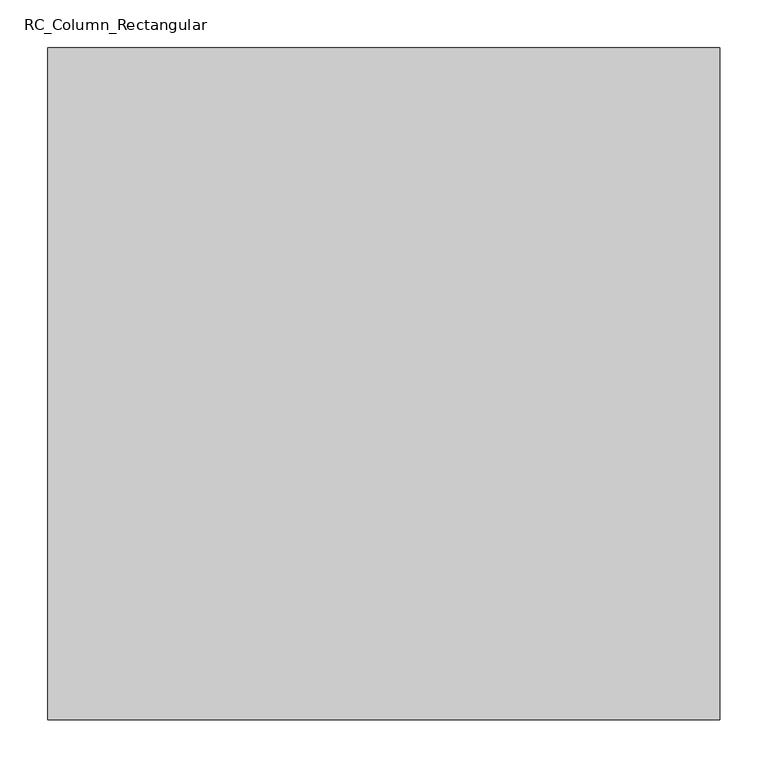
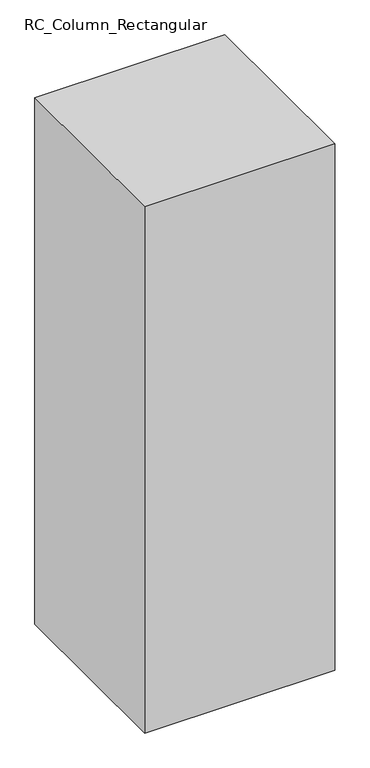
"""IFC4 building model written with IfcOpenShell, lengths in millimetres: column geometry, RC_Column_Rectangular : H_SC_AR_S15_UG PED_W700xL700_Bit_PD3."""

import ifcopenshell
import ifcopenshell.guid

model = None  # the IFC model being written
_history = None  # IfcOwnerHistory: only IFC2X3 demands one
_inside = {}  # id of a spatial element -> (the spatial element, [elements in it])
_under = {}  # id of a project, library or spatial element -> (it, [spatial elements below it])
_declared = {}  # id of a project -> (the project, [libraries it declares])
_typed = {}  # id of a type object -> (the type object, [elements of that type])
_made_of = {}  # id of a material, layer set ... -> (it, [elements and type objects made of it])


def new_model(schema):
    """Start an empty IFC model of exactly this schema.

    Asked for "IFC4X3", IfcOpenShell would pick the latest addendum, in which some entities
    have other attributes; the version numbers below select the first issue.
    IFC2X3 requires an IfcOwnerHistory on every rooted entity: one is made here for all.
    """
    global model, _history
    if schema == "IFC4X3":
        model = ifcopenshell.file(schema_version=(4, 3, 0, 0))
    else:
        model = ifcopenshell.file(schema=schema)
    _inside.clear()
    _under.clear()
    _declared.clear()
    _typed.clear()
    _made_of.clear()
    _history = None
    if model.schema == "IFC2X3":
        org = make("IfcOrganization", Name="unknown")
        user = make(
            "IfcPersonAndOrganization",
            ThePerson=make("IfcPerson", FamilyName="unknown"),
            TheOrganization=org,
        )
        app = make(
            "IfcApplication",
            ApplicationDeveloper=org,
            Version="unknown",
            ApplicationFullName="unknown",
            ApplicationIdentifier="unknown",
        )
        _history = make(
            "IfcOwnerHistory",
            OwningUser=user,
            OwningApplication=app,
            ChangeAction="ADDED",
            CreationDate=0,
        )
    return model


def make(cls, **values):
    """One entity of the class cls with the attributes given. An attribute that is None is left unset."""
    return model.create_entity(
        cls, **{name: value for name, value in values.items() if value is not None}
    )


def rooted(cls, **values):
    """An entity with a GlobalId (a new one), such as an element, a storey or a relation."""
    return make(cls, GlobalId=ifcopenshell.guid.new(), OwnerHistory=_history, **values)


def si_unit(unit_type, name, prefix=None):
    """IfcSIUnit, for example si_unit("LENGTHUNIT", "METRE", prefix="MILLI")."""
    return make("IfcSIUnit", UnitType=unit_type, Prefix=prefix, Name=name)


def assignment(units):
    """IfcUnitAssignment: the units of a project."""
    return None if units is None else make("IfcUnitAssignment", Units=units)


def point(xyz):
    """IfcCartesianPoint."""
    return None if xyz is None else make("IfcCartesianPoint", Coordinates=xyz)


def direction(xyz):
    """IfcDirection."""
    return None if xyz is None else make("IfcDirection", DirectionRatios=xyz)


def frame(location, z_axis=None, x_axis=None):
    """IfcAxis2Placement3D, a coordinate frame: its origin and axes. An axis left out is left unset."""
    return make(
        "IfcAxis2Placement3D",
        Location=point(location),
        Axis=direction(z_axis),
        RefDirection=direction(x_axis),
    )


def origin():
    """The frame at (0, 0, 0) with its axes left unset."""
    return frame((0.0, 0.0, 0.0))


def place(relative_to, where):
    """IfcLocalPlacement: puts the frame where relative to a parent placement (None: the world)."""
    return make(
        "IfcLocalPlacement", PlacementRelTo=relative_to, RelativePlacement=where
    )


def context(
    kind, dimensions, precision=None, world=None, true_north=None, identifier=None
):
    """IfcGeometricRepresentationContext, for example the 3D "Model" context."""
    return make(
        "IfcGeometricRepresentationContext",
        ContextIdentifier=identifier,
        ContextType=kind,
        CoordinateSpaceDimension=dimensions,
        Precision=precision,
        WorldCoordinateSystem=world,
        TrueNorth=true_north,
    )


def project(units=None, contexts=None):
    """IfcProject with its units and contexts."""
    return rooted(
        "IfcProject",
        Name="project",
        RepresentationContexts=contexts,
        UnitsInContext=assignment(units),
    )


def spatial(cls, under=None, at=None, **own):
    """A site, building, storey or space (cls), placed at a placement, below another one or the project."""
    s = rooted(cls, ObjectPlacement=at, **own)
    if under is not None:
        _under.setdefault(under.id(), (under, []))[1].append(s)
    return s


def polyline(points):
    """IfcPolyline through the points."""
    return make("IfcPolyline", Points=[point(p) for p in points])


def outline(outer, holes=None, kind="AREA"):
    """IfcArbitraryClosedProfileDef: a profile drawn as a closed curve; with holes, ...WithVoids."""
    if holes is None:
        return make("IfcArbitraryClosedProfileDef", ProfileType=kind, OuterCurve=outer)
    return make(
        "IfcArbitraryProfileDefWithVoids",
        ProfileType=kind,
        OuterCurve=outer,
        InnerCurves=holes,
    )


def extrude(swept, where, along, depth):
    """IfcExtrudedAreaSolid: the profile swept, set in the frame where, extruded along a direction by depth."""
    return make(
        "IfcExtrudedAreaSolid",
        SweptArea=swept,
        Position=where,
        ExtrudedDirection=direction(along),
        Depth=depth,
    )


def shape(context_of_items, identifier, shape_type, items):
    """IfcShapeRepresentation: the items that make up one representation, for example the "Body"."""
    return make(
        "IfcShapeRepresentation",
        ContextOfItems=context_of_items,
        RepresentationIdentifier=identifier,
        RepresentationType=shape_type,
        Items=items,
    )


def source(mapping_origin, context_of_items, identifier, shape_type, items):
    """IfcRepresentationMap: a shape defined once, which mapped items show again and again."""
    return make(
        "IfcRepresentationMap",
        MappingOrigin=mapping_origin,
        MappedRepresentation=shape(context_of_items, identifier, shape_type, items),
    )


def transform(
    local_origin,
    x_axis=None,
    y_axis=None,
    z_axis=None,
    scale=None,
    scale2=None,
    scale3=None,
    uniform=True,
):
    """IfcCartesianTransformationOperator3D, or its non-uniform kind. x_axis, y_axis, z_axis: its Axis1, 2, 3."""
    if uniform:
        return make(
            "IfcCartesianTransformationOperator3D",
            Axis1=direction(x_axis),
            Axis2=direction(y_axis),
            LocalOrigin=point(local_origin),
            Scale=scale,
            Axis3=direction(z_axis),
        )
    return make(
        "IfcCartesianTransformationOperator3DnonUniform",
        Axis1=direction(x_axis),
        Axis2=direction(y_axis),
        LocalOrigin=point(local_origin),
        Scale=scale,
        Axis3=direction(z_axis),
        Scale2=scale2,
        Scale3=scale3,
    )


def mapped(mapping_source, mapping_target):
    """IfcMappedItem: shows the shape of a source again, moved by a transform."""
    return make(
        "IfcMappedItem", MappingSource=mapping_source, MappingTarget=mapping_target
    )


def made_of(thing, what):
    """Note that an element or type object is made of a material, layer set ...; save() writes the relation."""
    if what is not None:
        _made_of.setdefault(what.id(), (what, []))[1].append(thing)
    return thing


def element(
    cls,
    number,
    at=None,
    inside=None,
    cuts=None,
    type_object=None,
    material=None,
    context=None,
    identifier="Body",
    shape_type=None,
    held_by="IfcProductDefinitionShape",
    body=None,
    shapes=None,
    **own,
):
    """One element of the class cls, such as IfcWall. Its Tag is "e" and its number.

    at: its placement. inside: the storey or other place that contains it. cuts: it is an
    opening in that element (IfcRelVoidsElement). A single representation is given by context,
    identifier, shape_type and body (its items); several are given by shapes. held_by: the class
    of the entity that holds the representations. save() writes the other relations.
    """
    e = rooted(cls, Tag="e%d" % number, ObjectPlacement=at, **own)
    if body is not None:
        shapes = [shape(context, identifier, shape_type, body)]
    if shapes is not None:
        e.Representation = make(held_by, Representations=shapes)
    if inside is not None:
        _inside.setdefault(inside.id(), (inside, []))[1].append(e)
    if cuts is not None:
        rooted(
            "IfcRelVoidsElement", RelatingBuildingElement=cuts, RelatedOpeningElement=e
        )
    if type_object is not None:
        _typed.setdefault(type_object.id(), (type_object, []))[1].append(e)
    return made_of(e, material)


def aggregate(whole, parts):
    """IfcRelAggregates: a whole, such as a stair, and the parts it consists of."""
    return rooted("IfcRelAggregates", RelatingObject=whole, RelatedObjects=parts)


def save(model, path):
    """Write the relations noted so far, then the file.

    IfcRelAggregates (storeys below a building ...), IfcRelContainedInSpatialStructure (elements
    in a storey), IfcRelDefinesByType, IfcRelAssociatesMaterial and IfcRelDeclares: one each for
    every whole, place, type object, material and project.
    """
    for whole, parts in _under.values():
        aggregate(whole, parts)
    for where, things in _inside.values():
        rooted(
            "IfcRelContainedInSpatialStructure",
            RelatedElements=things,
            RelatingStructure=where,
        )
    for kind, things in _typed.values():
        rooted("IfcRelDefinesByType", RelatedObjects=things, RelatingType=kind)
    for what, things in _made_of.values():
        rooted("IfcRelAssociatesMaterial", RelatedObjects=things, RelatingMaterial=what)
    for by, libraries in _declared.values():
        rooted("IfcRelDeclares", RelatingContext=by, RelatedDefinitions=libraries)
    model.write(path)


def rc_column_rectangular_f0532c4b(model_context):
    return source(origin(), model_context, "Body", "SweptSolid", [
        extrude(outline(polyline([(350.0, 350.0), (350.0, -350.0), (-350.0, -350.0), (-350.0, 350.0), (350.0, 350.0)])), frame((0.0, 0.0, -9380.1756499), z_axis=(0.0, 0.0, 1.0), x_axis=(1.0, 0.0, 0.0)), (0.0, 0.0, 1.0), 2050.0),
    ])


if __name__ == "__main__":
    model = new_model("IFC4")
    model_context = context("Model", 3, world=origin())
    ifc_project = project(units=[si_unit("LENGTHUNIT", "METRE", prefix="MILLI")], contexts=[model_context])
    site = spatial("IfcSite", under=ifc_project)
    building = spatial("IfcBuilding", under=site)
    placement = place(None, origin())
    rc_column_rectangular_shape = rc_column_rectangular_f0532c4b(model_context)
    element("IfcColumn", 1, ObjectType="RC_Column_Rectangular : H_SC_AR_S15_UG PED_W700xL700_Bit_PD3", at=placement, inside=building, context=model_context, shape_type="MappedRepresentation", body=[
        mapped(rc_column_rectangular_shape, transform((0.0, 0.0, 0.0), x_axis=(1.0, 0.0, 0.0), y_axis=(0.0, 1.0, 0.0), z_axis=(0.0, 0.0, 1.0))),
    ])
    save(model, "model.ifc")

# Revit data of these elements
# Type "RC_Column_Rectangular : H_SC_AR_S15_UG PED_W700xL700_Bit_PD3"
#   Type Mark = "PD3"
#   Width = 700 mm
#   Length = 700 mm
#   hec_material3 [instance default] = none
#   hec_material2 [instance default] = none
#   hec_material1 [instance default] = none
#   Structural Material [instance default] = none
#   Description = (empty or 0)
